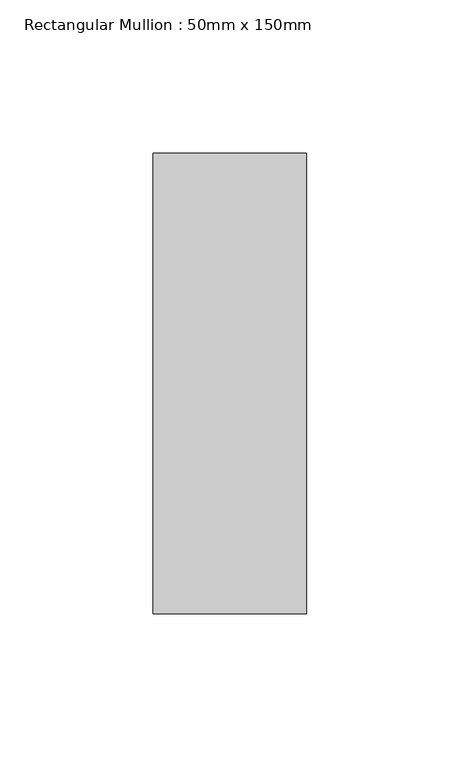
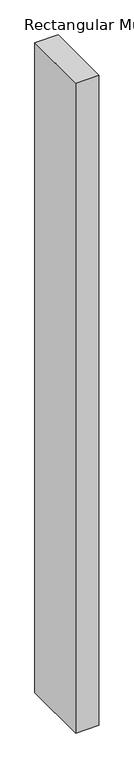
"""IFC4 building model written with IfcOpenShell, lengths in millimetres: member geometry, Rectangular Mullion : 50mm x 150mm."""

from ifc_helpers import new_model, si_unit, frame, origin, place, context, project, spatial, polyline, outline, extrude, source, transform, mapped, element, save


def rectangular_mullion_50mm_x_150mm_1758c09b(model_context):
    return source(origin(), model_context, "Body", "SweptSolid", [
        extrude(outline(polyline([(0.0, 75.0), (0.0, -75.0), (-50.0, -75.0), (-50.0, 75.0), (0.0, 75.0)])), frame((0.0, 0.0, -1465.8166232), z_axis=(0.0, 0.0, 1.0), x_axis=(1.0, 0.0, 0.0)), (0.0, 0.0, 1.0), 1465.8166232),
    ])


if __name__ == "__main__":
    model = new_model("IFC4")
    model_context = context("Model", 3, world=origin())
    ifc_project = project(units=[si_unit("LENGTHUNIT", "METRE", prefix="MILLI")], contexts=[model_context])
    site = spatial("IfcSite", under=ifc_project)
    building = spatial("IfcBuilding", under=site)
    placement = place(None, origin())
    rectangular_mullion_50mm_x_150mm_shape = rectangular_mullion_50mm_x_150mm_1758c09b(model_context)
    element("IfcMember", 1, ObjectType="Rectangular Mullion : 50mm x 150mm", at=placement, inside=building, context=model_context, shape_type="MappedRepresentation", body=[
        mapped(rectangular_mullion_50mm_x_150mm_shape, transform((0.0, 0.0, 0.0), x_axis=(1.0, 0.0, 0.0), y_axis=(0.0, 1.0, 0.0), z_axis=(0.0, 0.0, 1.0))),
    ])
    save(model, "model.ifc")

# Revit data of these elements
# Type "Rectangular Mullion : 50mm x 150mm"
#   built-in parameter 1007304 = 0.492126 (stored number, unit not read)
#   built-in parameter 1007301 = 0.082021 (stored number, unit not read)
#   built-in parameter 1007300 = 0.082021 (stored number, unit not read)
# Element 1 (IfcMember, "Rectangular Mullion : 50mm x 150mm")
#   Materials on its faces: "Aluminum"
# Materials
#   "Aluminum": class "Metal", colour RGB 244 244 244, transparency 0, Description = "Aluminum 6061", Cost = 0
